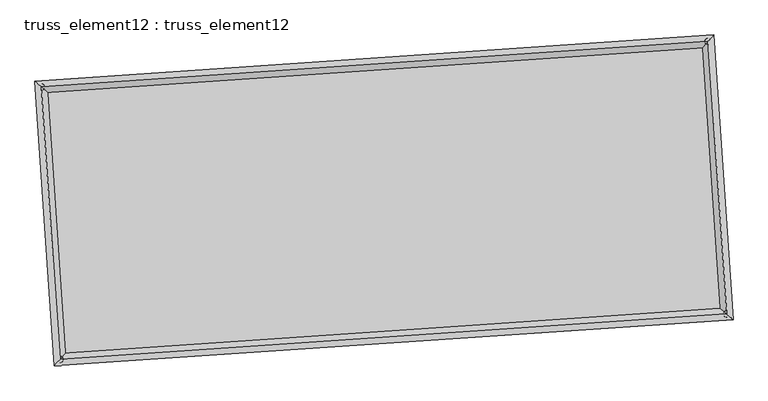
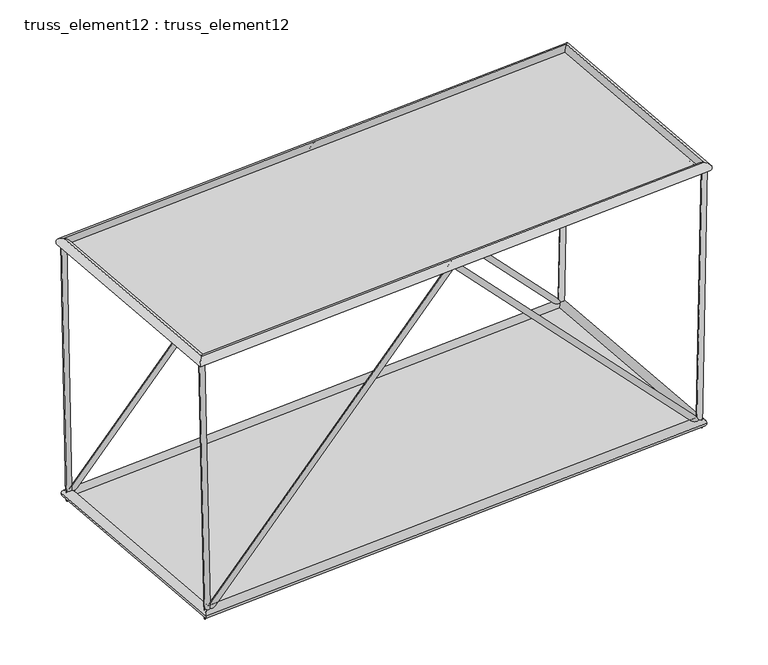
"""IFC4 building model written with IfcOpenShell, lengths in millimetres: plate geometry, truss_element12 : truss_element12."""

from ifc_helpers import new_model, si_unit, frame, origin, origin_with_axes, place, context, project, spatial, polyline, circle_curve, ellipse_curve, outline, extrude, source, transform, mapped, element, save
from ifc_brep_helpers import plane_surface, cylinder_surface, advanced_brep


def truss_element12_truss_element12_b131e6b3(model_context):
    return source(origin(), model_context, "Body", "SolidModel", [
        advanced_brep(
        [(-3768.4426764, 2269.1666348, 4999.9589336), (-3867.5246147, 2255.8068381, 4997.8888311), (-3667.4480193, 2276.0530765, 121.5783447), (-3761.5388635, 2263.0336036, -121.5783447), (1063.0770133, 2598.6095961, 5071.0530229), (1063.5348076, 2592.0370354, 4926.8211016), (5794.8562778, 2921.251637, 121.5871066), (5889.9046992, 2921.1288515, -121.5871066), (5894.6060324, 2928.0531935, 4999.9725392), (5994.5849006, 2928.2665965, 4997.9279449)],
        [
            (0, 1, circle_curve(frame((-3817.9836456, 2262.4867364, 4998.9238824), z_axis=(-0.02069804082979307, -0.0014113207235644356, 0.9997847764792298), x_axis=(-0.1335984293387775, 0.9910346065567788, -0.0013668522459998886)), 50.0)),
            (1, 0, circle_curve(frame((-3817.9836456, 2262.4867364, 4998.9238824), z_axis=(-0.02069804082979307, -0.0014113207235644356, 0.9997847764792298), x_axis=(-0.1335984293387775, 0.9910346065567788, -0.0013668522459998886)), 50.0)),
            (0, 2),
            (2, 3, ellipse_curve(frame((-3714.4934414, 2269.54334, 0.0), z_axis=(-0.9295901312719013, -0.06338521734851928, 0.3631039824397008), x_axis=(0.3622628143287531, 0.024701324219198188, 0.9317486237910038)), 130.7681897, 50.0)),
            (3, 1),
            (3, 2, ellipse_curve(frame((-3714.4934414, 2269.54334, 0.0), z_axis=(-0.9295901312719013, -0.06338521734851928, 0.3631039824397008), x_axis=(0.3622628143287531, 0.024701324219198188, 0.9317486237910038)), 130.7681897, 50.0)),
            (2, 4),
            (4, 5, ellipse_curve(frame((1063.3059105, 2595.3233157, 4998.9370622), z_axis=(-0.9976833938584647, -0.06802823807757281, -6.665670624892205e-05), x_axis=(6.650228906150557e-05, 4.534538292236935e-06, -0.9999999977784416)), 72.2729929, 50.0)),
            (5, 3),
            (5, 4, ellipse_curve(frame((1063.3059105, 2595.3233157, 4998.9370622), z_axis=(-0.9976833938584647, -0.06802823807757281, -6.665670624892205e-05), x_axis=(6.650228906150557e-05, 4.534538292236935e-06, -0.9999999977784416)), 72.2729929, 50.0)),
            (4, 6),
            (6, 7, ellipse_curve(frame((5842.3804885, 2921.1902443, 0.0), z_axis=(-0.9295196526265941, -0.06338041167761001, -0.3632852031070254), x_axis=(-0.3624436151795683, -0.024713652341926975, 0.9316779814954775)), 130.7875297, 50.0)),
            (7, 5),
            (7, 6, ellipse_curve(frame((5842.3804885, 2921.1902443, 0.0), z_axis=(-0.9295196526265941, -0.06338041167761001, -0.3632852031070254), x_axis=(-0.3624436151795683, -0.024713652341926975, 0.9316779814954775)), 130.7875297, 50.0)),
            (8, 9, circle_curve(frame((5944.5954665, 2928.159895, 4998.950242), z_axis=(0.02044299559371984, 0.0013939301584341597, 0.9997900484050983), x_axis=(-0.0021620821975439704, 0.9999967514320084, -0.001350009629994563)), 50.0)),
            (9, 8, circle_curve(frame((5944.5954665, 2928.159895, 4998.950242), z_axis=(0.02044299559371984, 0.0013939301584341597, 0.9997900484050983), x_axis=(-0.0021620821975439704, 0.9999967514320084, -0.001350009629994563)), 50.0)),
            (6, 8),
            (9, 7),
        ],
        [
            plane_surface(frame((-3817.9836456, 2312.4866866, 4998.9944636), z_axis=(-0.02069804082979222, -0.0014113207235603269, 0.9997847764792298), x_axis=(0.999785772606216, -2.9217833220407372e-05, 0.020698020207497326))),
            cylinder_surface(frame((-3817.9836456, 2262.4867364, 4998.9238824), z_axis=(-0.02069804082979307, -0.0014113207235644356, 0.9997847764792298), x_axis=(-0.1335984293387775, 0.9910346065567788, -0.0013668522459998886)), 50.0),
            cylinder_surface(frame((-3714.4934414, 2269.54334, 0.0), z_axis=(-0.6901706602776504, -0.047060113740035145, -0.7221148145459193), x_axis=(-0.02041427160093359, 0.9987522040196589, -0.04557732419610876)), 50.0),
            cylinder_surface(frame((1063.3059105, 2595.3233157, 4998.9370622), z_axis=(-0.6902666987206849, -0.04706666223638937, 0.7220225854799648), x_axis=(-0.11534052405583756, 0.9922795437132268, -0.04558366635972915)), 50.0),
            plane_surface(frame((5944.5954665, 2878.1599436, 4999.0199531), z_axis=(0.020442995593722254, 0.0013939301584386188, 0.9997900484050981), x_axis=(0.9997910201292843, -2.850206444371398e-05, -0.020442975724616754))),
            cylinder_surface(frame((5842.3804885, 2921.1902443, 0.0), z_axis=(-0.020442995593719836, -0.0013939301584341595, -0.9997900484050981), x_axis=(-0.0021620821975439704, 0.9999967514320084, -0.001350009629994563)), 50.0),
        ],
        [
            (0, [[1, 2]]),
            (1, [[-1, 3, 4, 5]]),
            (1, [[-2, -5, 6, -3]]),
            (2, [[-4, 7, 8, 9]]),
            (2, [[-6, -9, 10, -7]]),
            (3, [[-8, 11, 12, 13]]),
            (3, [[-10, -13, 14, -11]]),
            (4, [[15, 16]]),
            (5, [[-12, 17, -16, 18]]),
            (5, [[-14, -18, -15, -17]]),
        ],
    ),
        advanced_brep(
        [(-3496.3297235, -1721.5669495, 4999.9589336), (-3595.4116618, -1734.9267462, 4997.8888311), (-3395.3350664, -1714.6805078, 121.5783447), (-3489.4259106, -1727.6999807, -121.5783447), (1335.1899662, -1392.1239882, 5071.0530229), (1335.6477605, -1398.6965489, 4926.8211016), (6066.9692307, -1069.4819473, 121.5871066), (6162.0176521, -1069.6047328, -121.5871066), (6166.7189853, -1062.6803908, 4999.9725392), (6266.6978535, -1062.4669878, 4997.9279449)],
        [
            (0, 1, circle_curve(frame((-3545.8706927, -1728.2468479, 4998.9238824), z_axis=(-0.02069804082979312, -0.001411320723564435, 0.9997847764792299), x_axis=(-0.1335984293387778, 0.9910346065567789, -0.001366852245999902)), 50.0)),
            (1, 0, circle_curve(frame((-3545.8706927, -1728.2468479, 4998.9238824), z_axis=(-0.02069804082979312, -0.001411320723564435, 0.9997847764792299), x_axis=(-0.1335984293387778, 0.9910346065567789, -0.001366852245999902)), 50.0)),
            (0, 2),
            (2, 3, ellipse_curve(frame((-3442.3804885, -1721.1902443, 0.0), z_axis=(-0.929590131271901, -0.06338521734851939, 0.36310398243970093), x_axis=(0.36226281432875324, 0.024701324219198247, 0.9317486237910038)), 130.7681897, 50.0)),
            (3, 1),
            (3, 2, ellipse_curve(frame((-3442.3804885, -1721.1902443, 0.0), z_axis=(-0.929590131271901, -0.06338521734851939, 0.36310398243970093), x_axis=(0.36226281432875324, 0.024701324219198247, 0.9317486237910038)), 130.7681897, 50.0)),
            (2, 4),
            (4, 5, ellipse_curve(frame((1335.4188634, -1395.4102686, 4998.9370622), z_axis=(-0.9976833938584647, -0.06802823807757304, -6.665670624852088e-05), x_axis=(6.650228906104429e-05, 4.5345382922849825e-06, -0.9999999977784416)), 72.2729929, 50.0)),
            (5, 3),
            (5, 4, ellipse_curve(frame((1335.4188634, -1395.4102686, 4998.9370622), z_axis=(-0.9976833938584647, -0.06802823807757304, -6.665670624852088e-05), x_axis=(6.650228906104429e-05, 4.5345382922849825e-06, -0.9999999977784416)), 72.2729929, 50.0)),
            (4, 6),
            (6, 7, ellipse_curve(frame((6114.4934414, -1069.54334, 0.0), z_axis=(-0.9295196526265943, -0.06338041167761027, -0.3632852031070244), x_axis=(-0.3624436151795674, -0.02471365234192704, 0.9316779814954779)), 130.7875297, 50.0)),
            (7, 5),
            (7, 6, ellipse_curve(frame((6114.4934414, -1069.54334, 0.0), z_axis=(-0.9295196526265943, -0.06338041167761027, -0.3632852031070244), x_axis=(-0.3624436151795674, -0.02471365234192704, 0.9316779814954779)), 130.7875297, 50.0)),
            (8, 9, circle_curve(frame((6216.7084194, -1062.5736893, 4998.950242), z_axis=(0.020442995593720842, 0.0013939301584342109, 0.9997900484050981), x_axis=(-0.002162082197543998, 0.9999967514320084, -0.0013500096299946115)), 50.0)),
            (9, 8, circle_curve(frame((6216.7084194, -1062.5736893, 4998.950242), z_axis=(0.020442995593720842, 0.0013939301584342109, 0.9997900484050981), x_axis=(-0.002162082197543998, 0.9999967514320084, -0.0013500096299946115)), 50.0)),
            (6, 8),
            (9, 7),
        ],
        [
            plane_surface(frame((-3545.8706927, -1678.2468977, 4998.9944636), z_axis=(-0.020698040829792222, -0.0014113207235603234, 0.9997847764792299), x_axis=(0.999785772606216, -2.9217833220407372e-05, 0.020698020207497326))),
            cylinder_surface(frame((-3545.8706927, -1728.2468479, 4998.9238824), z_axis=(-0.020698040829793124, -0.0014113207235644351, 0.9997847764792301), x_axis=(-0.1335984293387778, 0.9910346065567789, -0.001366852245999902)), 50.0),
            cylinder_surface(frame((-3442.3804885, -1721.1902443, 0.0), z_axis=(-0.6901706602776506, -0.047060113740035256, -0.7221148145459192), x_axis=(-0.020414271600933634, 0.9987522040196589, -0.04557732419610887)), 50.0),
            cylinder_surface(frame((1335.4188634, -1395.4102686, 4998.9370622), z_axis=(-0.6902666987206844, -0.04706666223638954, 0.7220225854799652), x_axis=(-0.115340524055838, 0.9922795437132268, -0.0455836663597292)), 50.0),
            plane_surface(frame((6216.7084194, -1112.5736407, 4999.0199531), z_axis=(0.020442995593722254, 0.0013939301584386132, 0.9997900484050981), x_axis=(0.9997910201292843, -2.8502064444602157e-05, -0.020442975724616754))),
            cylinder_surface(frame((6114.4934414, -1069.54334, 0.0), z_axis=(-0.020442995593720842, -0.0013939301584342109, -0.9997900484050981), x_axis=(-0.002162082197543998, 0.9999967514320084, -0.0013500096299946115)), 50.0),
        ],
        [
            (0, [[1, 2]]),
            (1, [[-1, 3, 4, 5]]),
            (1, [[-2, -5, 6, -3]]),
            (2, [[-4, 7, 8, 9]]),
            (2, [[-6, -9, 10, -7]]),
            (3, [[-8, 11, 12, 13]]),
            (3, [[-10, -13, 14, -11]]),
            (4, [[15, 16]]),
            (5, [[-12, 17, -16, 18]]),
            (5, [[-14, -18, -15, -17]]),
        ],
    ),
        advanced_brep(
        [(-3545.8638321, -1728.2392441, 4908.9238827), (-3545.8775532, -1728.2544517, 5088.9238821), (-3817.9914747, 2262.4933386, 5088.9238821), (-3817.9758164, 2262.4801343, 4908.9238827), (5944.6018432, 2928.1674658, 5088.9502418), (5944.5890897, 2928.1523242, 4908.9502423), (6216.7157648, -1062.5803244, 5088.9502418), (6216.701074, -1062.5670541, 4908.9502423)],
        [
            (0, 1, ellipse_curve(frame((-3545.8706927, -1728.2468479, 4998.9238824), z_axis=(-0.7535719234028934, 0.657365466278261, -1.9048135840263405e-06), x_axis=(-0.6573654662755266, -0.7535719234052785, -1.904813584026813e-06)), 127.2792206, 90.0)),
            (1, 2),
            (2, 3, ellipse_curve(frame((-3817.9836456, 2262.4867364, 4998.9238824), z_axis=(-0.6573654662755267, -0.7535719234052785, -1.904813584027251e-06), x_axis=(0.7535719234028933, -0.6573654662782611, 1.9048135840267782e-06)), 127.2792206, 90.0)),
            (3, 0),
            (1, 0, ellipse_curve(frame((-3545.8706927, -1728.2468479, 4998.9238824), z_axis=(-0.7535719234028934, 0.657365466278261, -1.9048135840263405e-06), x_axis=(-0.6573654662755266, -0.7535719234052785, -1.904813584026813e-06)), 127.2792206, 90.0)),
            (3, 2, ellipse_curve(frame((-3817.9836456, 2262.4867364, 4998.9238824), z_axis=(-0.6573654662755267, -0.7535719234052785, -1.904813584027251e-06), x_axis=(0.7535719234028933, -0.6573654662782611, 1.9048135840267782e-06)), 127.2792206, 90.0)),
            (2, 4),
            (4, 5, ellipse_curve(frame((5944.5954665, 2928.159895, 4998.950242), z_axis=(-0.753571923402893, 0.6573654662782614, -1.904813584027219e-06), x_axis=(-0.6573654662755272, -0.7535719234052781, -1.9048135840268106e-06)), 127.2792206, 90.0)),
            (5, 3),
            (5, 4, ellipse_curve(frame((5944.5954665, 2928.159895, 4998.950242), z_axis=(-0.753571923402893, 0.6573654662782614, -1.904813584027219e-06), x_axis=(-0.6573654662755272, -0.7535719234052781, -1.9048135840268106e-06)), 127.2792206, 90.0)),
            (4, 6),
            (6, 7, ellipse_curve(frame((6216.7084194, -1062.5736893, 4998.950242), z_axis=(0.6573654662755272, 0.7535719234052781, 1.9048135840263727e-06), x_axis=(-0.7535719234028929, 0.6573654662782614, -1.9048135840267807e-06)), 127.2792206, 90.0)),
            (7, 5),
            (7, 6, ellipse_curve(frame((6216.7084194, -1062.5736893, 4998.950242), z_axis=(0.6573654662755272, 0.7535719234052781, 1.9048135840263727e-06), x_axis=(-0.7535719234028929, 0.6573654662782614, -1.9048135840267807e-06)), 127.2792206, 90.0)),
            (6, 1),
            (0, 7),
        ],
        [
            cylinder_surface(frame((-3545.8706927, -1728.2468479, 4998.9238824), z_axis=(0.06802823822869399, -0.9976833960748771, 0.0), x_axis=(-0.9976833927370898, -0.06802823800110296, -8.179899131153941e-05)), 90.0),
            cylinder_surface(frame((-3817.9836456, 2262.4867364, 4998.9238824), z_axis=(-0.9976833960712572, -0.06802823822844672, -2.6938132043235077e-06), x_axis=(-0.06802823780324489, 0.9976833929678072, -7.910517811564465e-05)), 90.0),
            cylinder_surface(frame((5944.5954665, 2928.159895, 4998.950242), z_axis=(-0.068028238228693, 0.9976833960748774, 0.0), x_axis=(0.9976833931622919, 0.06802823803009488, -7.64113649197499e-05)), 90.0),
            cylinder_surface(frame((6216.7084194, -1062.5736893, 4998.950242), z_axis=(0.9976833960712573, 0.06802823822844663, 2.6938132043228885e-06), x_axis=(0.06802823822844663, -0.9976833929388144, -7.910517811564467e-05)), 90.0),
        ],
        [
            (0, [[1, 2, 3, 4]]),
            (0, [[5, -4, 6, -2]]),
            (1, [[-3, 7, 8, 9]]),
            (1, [[-6, -9, 10, -7]]),
            (2, [[-8, 11, 12, 13]]),
            (2, [[-10, -13, 14, -11]]),
            (3, [[-12, 15, -1, 16]]),
            (3, [[-14, -16, -5, -15]]),
        ],
    ),
        advanced_brep(
        [(-3358.7115243, -1625.2761972, 0.0), (-3526.0494527, -1817.1042913, 0.0), (-3810.4074885, 2353.2123043, 0.0), (-3618.5793943, 2185.8743758, 0.0), (5926.0494527, 3017.1042913, 0.0), (5758.7115243, 2825.2761972, 0.0), (6210.4074885, -1153.2123043, 0.0), (6018.5793943, -985.8743758, 0.0)],
        [
            (0, 1, ellipse_curve(frame((-3442.3804885, -1721.1902443, 0.0), z_axis=(-0.7535719234054582, 0.6573654662780803, 0.0), x_axis=(-0.6573654662780802, -0.7535719234054585, 0.0)), 127.2792206, 90.0)),
            (1, 2),
            (2, 3, ellipse_curve(frame((-3714.4934414, 2269.54334, 0.0), z_axis=(-0.6573654662780803, -0.7535719234054583, 0.0), x_axis=(0.7535719234054582, -0.6573654662780803, 0.0)), 127.2792206, 90.0)),
            (3, 0),
            (1, 0, ellipse_curve(frame((-3442.3804885, -1721.1902443, 0.0), z_axis=(-0.7535719234054582, 0.6573654662780803, 0.0), x_axis=(-0.6573654662780802, -0.7535719234054585, 0.0)), 127.2792206, 90.0)),
            (3, 2, ellipse_curve(frame((-3714.4934414, 2269.54334, 0.0), z_axis=(-0.6573654662780803, -0.7535719234054583, 0.0), x_axis=(0.7535719234054582, -0.6573654662780803, 0.0)), 127.2792206, 90.0)),
            (2, 4),
            (4, 5, ellipse_curve(frame((5842.3804885, 2921.1902443, 0.0), z_axis=(-0.753571923405458, 0.6573654662780808, 0.0), x_axis=(-0.6573654662780808, -0.7535719234054579, 0.0)), 127.2792206, 90.0)),
            (5, 3),
            (5, 4, ellipse_curve(frame((5842.3804885, 2921.1902443, 0.0), z_axis=(-0.753571923405458, 0.6573654662780808, 0.0), x_axis=(-0.6573654662780808, -0.7535719234054579, 0.0)), 127.2792206, 90.0)),
            (4, 6),
            (6, 7, ellipse_curve(frame((6114.4934414, -1069.54334, 0.0), z_axis=(0.6573654662780809, 0.7535719234054578, 0.0), x_axis=(-0.7535719234054576, 0.657365466278081, 0.0)), 127.2792206, 90.0)),
            (7, 5),
            (7, 6, ellipse_curve(frame((6114.4934414, -1069.54334, 0.0), z_axis=(0.6573654662780809, 0.7535719234054578, 0.0), x_axis=(-0.7535719234054576, 0.657365466278081, 0.0)), 127.2792206, 90.0)),
            (6, 1),
            (0, 7),
        ],
        [
            cylinder_surface(frame((-3442.3804885, -1721.1902443, 0.0), z_axis=(0.06802823822870205, -0.9976833960748765, 0.0), x_axis=(-0.9976833960748765, -0.06802823822870205, 0.0)), 90.0),
            cylinder_surface(frame((-3714.4934414, 2269.54334, 0.0), z_axis=(-0.9976833960748765, -0.06802823822870166, 0.0), x_axis=(-0.06802823822870166, 0.9976833960748765, 0.0)), 90.0),
            cylinder_surface(frame((5842.3804885, 2921.1902443, 0.0), z_axis=(-0.06802823822870079, 0.9976833960748767, 0.0), x_axis=(0.9976833960748767, 0.06802823822870079, 0.0)), 90.0),
            cylinder_surface(frame((6114.4934414, -1069.54334, 0.0), z_axis=(0.9976833960748767, 0.06802823822870135, 0.0), x_axis=(0.06802823822870135, -0.9976833960748767, 0.0)), 90.0),
        ],
        [
            (0, [[1, 2, 3, 4]]),
            (0, [[5, -4, 6, -2]]),
            (1, [[-3, 7, 8, 9]]),
            (1, [[-6, -9, 10, -7]]),
            (2, [[-8, 11, 12, 13]]),
            (2, [[-10, -13, 14, -11]]),
            (3, [[-12, 15, -1, 16]]),
            (3, [[-14, -16, -5, -15]]),
        ],
    ),
        extrude(outline(polyline([(-3442.3804885, -1721.1902443), (-3714.4934414, 2269.54334), (5842.3804885, 2921.1902443), (6114.4934414, -1069.54334), (-3442.3804885, -1721.1902443)])), origin_with_axes(), (0.0, 0.0, 1.0), 20.0),
        extrude(outline(polyline([(-2000.0, 4892.6238276), (2000.0, 4892.6238276), (1999.9999999, -4892.6238276), (-2000.0000001, -4892.6238276), (-2000.0, 4892.6238276)])), frame((1199.3623869, 599.9565236, 4998.9370622), z_axis=(-2.6875727060805124e-06, -1.8325536640732116e-07, 0.9999999999963718), x_axis=(-0.06802823822870185, 0.9976833960748765, 0.0)), (0.0, 0.0, 1.0), 20.0),
    ])


if __name__ == "__main__":
    model = new_model("IFC4")
    model_context = context("Model", 3, world=origin())
    ifc_project = project(units=[si_unit("LENGTHUNIT", "METRE", prefix="MILLI")], contexts=[model_context])
    site = spatial("IfcSite", under=ifc_project)
    building = spatial("IfcBuilding", under=site)
    placement = place(None, origin())
    truss_element12_truss_element12_shape = truss_element12_truss_element12_b131e6b3(model_context)
    element("IfcPlate", 1, ObjectType="truss_element12 : truss_element12", at=placement, inside=building, context=model_context, shape_type="MappedRepresentation", body=[
        mapped(truss_element12_truss_element12_shape, transform((0.0, 0.0, 0.0), x_axis=(1.0, 0.0, 0.0), y_axis=(0.0, 1.0, 0.0), z_axis=(0.0, 0.0, 1.0))),
    ])
    save(model, "model.ifc")

# Revit data of these elements
# Type "truss_element12 : truss_element12"
#   steellbar1 = 90 mm
#   steelbar2 = 50 mm
#   offset1 = 5000 mm
#   M = Default Roof
# Element 1 (IfcPlate, "truss_element12 : truss_element12")
#   Materials on its faces: "Default Roof"
# Materials
#   "Default Roof": class "Miscellaneous", colour RGB 0 127 0, transparency 0, Comments = "Rendering appearance not upgraded Rendering appearance not upgraded ", Cost = 0
